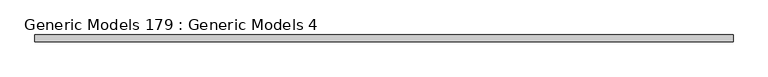
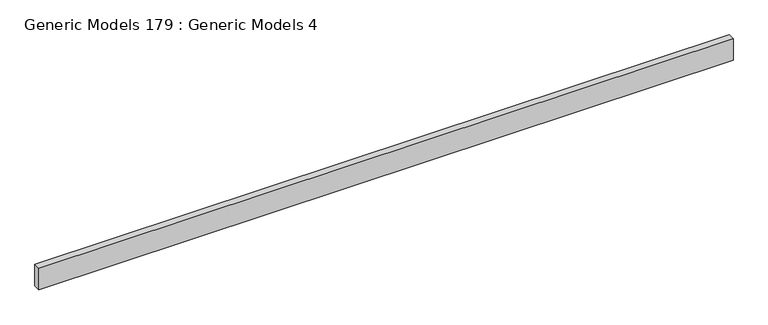
"""IFC4 building model written with IfcOpenShell, lengths in millimetres: proxy geometry, Generic Models 179 : Generic Models 4."""

from ifc_helpers import new_model, si_unit, frame, origin, place, context, project, spatial, polyline, outline, extrude, source, transform, mapped, element, save


def generic_models_179_generic_models_4_29f94ee0(model_context):
    return source(origin(), model_context, "Body", "SweptSolid", [
        extrude(outline(polyline([(2196.9263704, -5316.6308306), (2196.9263704, -5440.4558306), (-10256.7421316, -5440.4558306), (-10256.7421316, -5316.6308306), (2196.9263704, -5316.6308306)])), frame((0.0, 0.0, 126827.8280113), z_axis=(0.0, 0.0, 1.0), x_axis=(1.0, 0.0, 0.0)), (0.0, 0.0, 1.0), 406.4),
    ])


if __name__ == "__main__":
    model = new_model("IFC4")
    model_context = context("Model", 3, world=origin())
    ifc_project = project(units=[si_unit("LENGTHUNIT", "METRE", prefix="MILLI")], contexts=[model_context])
    site = spatial("IfcSite", under=ifc_project)
    building = spatial("IfcBuilding", under=site)
    placement = place(None, origin())
    generic_models_179_generic_models_4_shape = generic_models_179_generic_models_4_29f94ee0(model_context)
    element("IfcBuildingElementProxy", 1, Name="Generic Models 179 : Generic Models 4", ObjectType="Generic Models 179 : Generic Models 4", at=placement, inside=building, context=model_context, shape_type="MappedRepresentation", body=[
        mapped(generic_models_179_generic_models_4_shape, transform((0.0, 0.0, 0.0), x_axis=(1.0, 0.0, 0.0), y_axis=(0.0, 1.0, 0.0), z_axis=(0.0, 0.0, 1.0))),
    ])
    save(model, "model.ifc")

# Revit data of these elements
# Element 1 (IfcBuildingElementProxy, "Generic Models 179 : Generic Models 4")
#   Materials on its faces: "_BATT INSUL. (U-FACTOR = 0.065 MIN.) OVER CLASS II VAPOR RETARDER(TOWARD INTERIOR)"
# Materials
#   "_BATT INSUL. (U-FACTOR = 0.065 MIN.) OVER CLASS II VAPOR RETARDER(TOWARD INTERIOR)": class "Generic", colour RGB 227 210 251, transparency 0, Cost = 0
